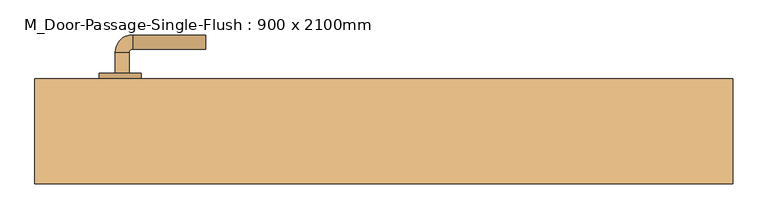
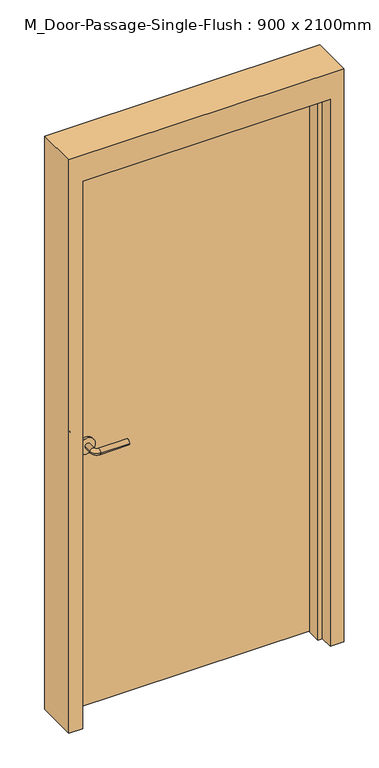
"""IFC4 building model written with IfcOpenShell, lengths in millimetres: door geometry, M_Door-Passage-Single-Flush : 900 x 2100mm."""

from ifc_helpers import new_model, si_unit, point, frame, frame_2d, origin, origin_with_axes, place, context, project, spatial, polyline, circle_curve, ellipse_curve, trimmed, segment, composite_curve, outline, extrude, faceted_brep, source, transform, mapped, element, save
from ifc_brep_helpers import plane_surface, cylinder_surface, revolved_surface, advanced_brep


def m_door_passage_single_flush_900_x_2100mm_f70d95c9(model_context):
    return source(origin(), model_context, "Body", "SolidModel", [
        advanced_brep(
        [(-384.990625, 3.35, 1000.0), (-364.990625, 3.35, 1000.0), (-364.990625, -26.65, 1000.0), (-384.990625, -26.65, 1000.0), (-359.990625, -31.65, 1000.0), (-359.990625, -51.65, 1000.0), (-254.990625, -51.65, 1000.0), (-254.990625, -31.65, 1000.0)],
        [
            (0, 1, circle_curve(frame((-374.990625, 3.35, 1000.0), z_axis=(0.0, 1.0, 0.0), x_axis=(1.0, 0.0, 0.0)), 10.0)),
            (1, 0, circle_curve(frame((-374.990625, 3.35, 1000.0), z_axis=(0.0, 1.0, 0.0), x_axis=(1.0, 0.0, 0.0)), 10.0)),
            (1, 2),
            (2, 3, circle_curve(frame((-374.990625, -26.65, 1000.0), z_axis=(0.0, 1.0, 0.0), x_axis=(1.0, 0.0, 0.0)), 10.0)),
            (3, 0),
            (3, 2, circle_curve(frame((-374.990625, -26.65, 1000.0), z_axis=(0.0, 1.0, 0.0), x_axis=(1.0, 0.0, 0.0)), 10.0)),
            (4, 5, circle_curve(frame((-359.990625, -41.65, 1000.0), z_axis=(-1.0, 0.0, 0.0), x_axis=(0.0, 1.0, 0.0)), 10.0)),
            (5, 3, circle_curve(frame((-359.990625, -26.65, 1000.0), z_axis=(0.0, 0.0, -1.0), x_axis=(-1.0, 0.0, 0.0)), 25.0)),
            (2, 4, circle_curve(frame((-359.990625, -26.65, 1000.0), z_axis=(0.0, 0.0, 1.0), x_axis=(-1.0, 0.0, 0.0)), 5.0)),
            (5, 4, circle_curve(frame((-359.990625, -41.65, 1000.0), z_axis=(-1.0, 0.0, 0.0), x_axis=(0.0, 1.0, 0.0)), 10.0)),
            (6, 7, circle_curve(frame((-254.990625, -41.65, 1000.0), z_axis=(1.0, 0.0, 0.0), x_axis=(0.0, 1.0, 0.0)), 10.0)),
            (7, 6, circle_curve(frame((-254.990625, -41.65, 1000.0), z_axis=(1.0, 0.0, 0.0), x_axis=(0.0, 1.0, 0.0)), 10.0)),
            (4, 7),
            (6, 5),
        ],
        [
            plane_surface(frame((-374.990625, 3.35, 1000.0), z_axis=(0.0, 1.0, 0.0), x_axis=(0.0, 0.0, 1.0))),
            cylinder_surface(frame((-374.990625, 3.35, 1000.0), z_axis=(0.0, 1.0, 0.0), x_axis=(1.0, 0.0, 0.0)), 10.0),
            revolved_surface(trimmed(ellipse_curve(frame((-374.990625, -26.65, 1000.0), z_axis=(0.0, -1.0, 0.0), x_axis=(1.0, 0.0, 0.0)), 10.0, 10.0), [point((-384.990625, -26.65, 1000.0))], [point((-364.990625, -26.65, 1000.0))], True, "CARTESIAN"), (-359.990625, -26.65, 1000.0), (0.0, 0.0, -1.0)),
            revolved_surface(trimmed(ellipse_curve(frame((-374.990625, -26.65, 1000.0), z_axis=(0.0, -1.0, 0.0), x_axis=(1.0, 0.0, 0.0)), 10.0, 10.0), [point((-364.990625, -26.65, 1000.0))], [point((-384.990625, -26.65, 1000.0))], True, "CARTESIAN"), (-359.990625, -26.65, 1000.0), (0.0, 0.0, -1.0)),
            plane_surface(frame((-254.990625, -41.65, 1000.0), z_axis=(1.0, 0.0, 0.0), x_axis=(0.0, 0.0, 1.0))),
            cylinder_surface(frame((-359.990625, -41.65, 1000.0), z_axis=(-1.0, 0.0, 0.0), x_axis=(0.0, 1.0, 0.0)), 10.0),
        ],
        [
            (0, [[1, 2]]),
            (1, [[3, 4, 5, -2]]),
            (1, [[-5, 6, -3, -1]]),
            (2, [[7, 8, -4, 9]]),
            (3, [[10, -9, -6, -8]]),
            (4, [[11, 12]]),
            (5, [[13, -11, 14, -7]]),
            (5, [[-14, -12, -13, -10]]),
        ],
    ),
        extrude(outline(composite_curve([segment(trimmed(circle_curve(frame_2d((1000.0, -377.490625)), 30.0), [point((1000.0, -407.490625))], [point((1000.0, -347.490625))], False, "CARTESIAN"), True, "CONTINUOUS"), segment(trimmed(circle_curve(frame_2d((1000.0, -377.490625)), 30.0), [point((1000.0, -347.490625))], [point((1000.0, -407.490625))], False, "CARTESIAN"), True, "CONTINUOUS")], self_intersect=False)), frame((0.0, 3.35, 0.0), z_axis=(0.0, 1.0, 0.0), x_axis=(0.0, 0.0, 1.0)), (0.0, 0.0, 1.0), 8.0),
        advanced_brep(
        [(-384.990625, 64.35, 1000.0), (-364.990625, 64.35, 1000.0), (-384.990625, 94.35, 1000.0), (-364.990625, 94.35, 1000.0), (-359.990625, 99.35, 1000.0), (-359.990625, 119.35, 1000.0), (-254.990625, 119.35, 1000.0), (-254.990625, 99.35, 1000.0)],
        [
            (0, 1, circle_curve(frame((-374.990625, 64.35, 1000.0), z_axis=(0.0, -1.0, 0.0), x_axis=(1.0, 0.0, 0.0)), 10.0)),
            (1, 0, circle_curve(frame((-374.990625, 64.35, 1000.0), z_axis=(0.0, -1.0, 0.0), x_axis=(1.0, 0.0, 0.0)), 10.0)),
            (0, 2),
            (2, 3, circle_curve(frame((-374.990625, 94.35, 1000.0), z_axis=(0.0, -1.0, 0.0), x_axis=(1.0, 0.0, 0.0)), 10.0)),
            (3, 1),
            (3, 2, circle_curve(frame((-374.990625, 94.35, 1000.0), z_axis=(0.0, -1.0, 0.0), x_axis=(1.0, 0.0, 0.0)), 10.0)),
            (4, 3, circle_curve(frame((-359.990625, 94.35, 1000.0), z_axis=(0.0, 0.0, 1.0), x_axis=(-1.0, 0.0, 0.0)), 5.0)),
            (2, 5, circle_curve(frame((-359.990625, 94.35, 1000.0), z_axis=(0.0, 0.0, -1.0), x_axis=(-1.0, 0.0, 0.0)), 25.0)),
            (5, 4, circle_curve(frame((-359.990625, 109.35, 1000.0), z_axis=(-1.0, 0.0, 0.0), x_axis=(0.0, -1.0, 0.0)), 10.0)),
            (4, 5, circle_curve(frame((-359.990625, 109.35, 1000.0), z_axis=(-1.0, 0.0, 0.0), x_axis=(0.0, -1.0, 0.0)), 10.0)),
            (6, 7, circle_curve(frame((-254.990625, 109.35, 1000.0), z_axis=(1.0, 0.0, 0.0), x_axis=(0.0, -1.0, 0.0)), 10.0)),
            (7, 6, circle_curve(frame((-254.990625, 109.35, 1000.0), z_axis=(1.0, 0.0, 0.0), x_axis=(0.0, -1.0, 0.0)), 10.0)),
            (5, 6),
            (7, 4),
        ],
        [
            plane_surface(frame((-374.990625, 64.35, 1000.0), z_axis=(0.0, -1.0, 0.0), x_axis=(0.0, 0.0, 1.0))),
            cylinder_surface(frame((-374.990625, 64.35, 1000.0), z_axis=(0.0, -1.0, 0.0), x_axis=(1.0, 0.0, 0.0)), 10.0),
            revolved_surface(trimmed(ellipse_curve(frame((-374.990625, 94.35, 1000.0), z_axis=(0.0, -1.0, 0.0), x_axis=(1.0, 0.0, 0.0)), 10.0, 10.0), [point((-384.990625, 94.35, 1000.0))], [point((-364.990625, 94.35, 1000.0))], True, "CARTESIAN"), (-359.990625, 94.35, 1000.0), (0.0, 0.0, -1.0)),
            revolved_surface(trimmed(ellipse_curve(frame((-374.990625, 94.35, 1000.0), z_axis=(0.0, -1.0, 0.0), x_axis=(1.0, 0.0, 0.0)), 10.0, 10.0), [point((-364.990625, 94.35, 1000.0))], [point((-384.990625, 94.35, 1000.0))], True, "CARTESIAN"), (-359.990625, 94.35, 1000.0), (0.0, 0.0, -1.0)),
            plane_surface(frame((-254.990625, 109.35, 1000.0), z_axis=(1.0, 0.0, 0.0), x_axis=(0.0, 0.0, 1.0))),
            cylinder_surface(frame((-359.990625, 109.35, 1000.0), z_axis=(-1.0, 0.0, 0.0), x_axis=(0.0, -1.0, 0.0)), 10.0),
        ],
        [
            (0, [[1, 2]]),
            (1, [[-1, 3, 4, 5]]),
            (1, [[-2, -5, 6, -3]]),
            (2, [[7, -4, 8, 9]]),
            (3, [[-8, -6, -7, 10]]),
            (4, [[11, 12]]),
            (5, [[-9, 13, -12, 14]]),
            (5, [[-10, -14, -11, -13]]),
        ],
    ),
        extrude(outline(composite_curve([segment(trimmed(circle_curve(frame_2d((1000.0, -377.490625)), 30.0), [point((1000.0, -407.490625))], [point((1000.0, -347.490625))], False, "CARTESIAN"), True, "CONTINUOUS"), segment(trimmed(circle_curve(frame_2d((1000.0, -377.490625)), 30.0), [point((1000.0, -347.490625))], [point((1000.0, -407.490625))], False, "CARTESIAN"), True, "CONTINUOUS")], self_intersect=False)), frame((0.0, 56.35, 0.0), z_axis=(0.0, 1.0, 0.0), x_axis=(0.0, 0.0, 1.0)), (0.0, 0.0, 1.0), 8.0),
        extrude(outline(polyline([(450.0, 11.35), (-450.0, 11.35), (-450.0, 56.35), (450.0, 56.35), (450.0, 11.35)])), origin_with_axes(), (0.0, 0.0, 1.0), 2100.0),
        faceted_brep([(450.0, 6.5875, 0.0), (450.0, 56.35, 0.0), (500.0, 56.35, 0.0), (500.0, -93.65, 0.0), (450.0, -93.65, 0.0), (450.0, -44.4375, 0.0), (434.125, -44.4375, 0.0), (434.125, 6.5875, 0.0), (450.0, 6.5875, 2100.0), (450.0, 56.35, 2100.0), (-450.0, 56.35, 2100.0), (-450.0, 56.35, 0.0), (-500.0, 56.35, 0.0), (-500.0, 56.35, 2200.0), (500.0, 56.35, 2200.0), (500.0, -93.65, 2200.0), (-500.0, -93.65, 2200.0), (-500.0, -93.65, 0.0), (-450.0, -93.65, 0.0), (-450.0, -93.65, 2100.0), (450.0, -93.65, 2100.0), (450.0, -44.4375, 2100.0), (-450.0, -44.4375, 2100.0), (-450.0, -44.4375, 0.0), (-434.125, -44.4375, 0.0), (-434.125, -44.4375, 2084.125), (434.125, -44.4375, 2084.125), (434.125, 6.5875, 2084.125), (-434.125, 6.5875, 2084.125), (-434.125, 6.5875, 0.0), (-450.0, 6.5875, 0.0), (-450.0, 6.5875, 2100.0)], [[[0, 1, 2, 3, 4, 5, 6, 7]], [[1, 0, 8, 9]], [[2, 1, 9, 10, 11, 12, 13, 14]], [[3, 2, 14, 15]], [[4, 3, 15, 16, 17, 18, 19, 20]], [[5, 4, 20, 21]], [[6, 5, 21, 22, 23, 24, 25, 26]], [[7, 6, 26, 27]], [[0, 7, 27, 28, 29, 30, 31, 8]], [[9, 8, 31, 10]], [[20, 19, 22, 21]], [[26, 25, 28, 27]], [[12, 11, 30, 29, 24, 23, 18, 17]], [[11, 10, 31, 30]], [[13, 12, 17, 16]], [[19, 18, 23, 22]], [[25, 24, 29, 28]], [[15, 14, 13, 16]]]),
    ])


if __name__ == "__main__":
    model = new_model("IFC4")
    model_context = context("Model", 3, world=origin())
    ifc_project = project(units=[si_unit("LENGTHUNIT", "METRE", prefix="MILLI")], contexts=[model_context])
    site = spatial("IfcSite", under=ifc_project)
    building = spatial("IfcBuilding", under=site)
    placement = place(None, origin())
    m_door_passage_single_flush_900_x_2100mm_shape = m_door_passage_single_flush_900_x_2100mm_f70d95c9(model_context)
    element("IfcDoor", 1, ObjectType="M_Door-Passage-Single-Flush : 900 x 2100mm", at=placement, inside=building, context=model_context, shape_type="MappedRepresentation", body=[
        mapped(m_door_passage_single_flush_900_x_2100mm_shape, transform((0.0, 0.0, 0.0), x_axis=(1.0, 0.0, 0.0), y_axis=(0.0, 1.0, 0.0), z_axis=(0.0, 0.0, 1.0))),
    ])
    save(model, "model.ifc")

# Revit data of these elements
# Type "M_Door-Passage-Single-Flush : 900 x 2100mm"
#   Type Mark = "38"
#   Analytic Construction = "Wooden"
#   Thickness = 45 mm
#   Thermal Resistance (R) = 0.455703 (m²·K)/W
#   Swing Angle [instance default] = 90.00°
#   Strike Height = 1000 mm
#   Rough Width [instance default] = 1000 mm
#   Rough Height [instance default] = 2200 mm
#   MF Opening Height [instance default] = 100 mm
#   MF Opening Width [instance default] = 100 mm
#   Inset Calculate [instance default] = 105 mm
#   Masonry Inset [instance default] = 25 mm
#   Height = 2100 mm
#   Width = 900 mm
#   Heat Transfer Coefficient (U) = 2.19465 W/(m²·K)
#   Masonry Frame Depth = 150 mm
#   Masonry Frame [instance default] = yes
#   Function = 1
#   Dry Wall Frame [instance default] = no
#   Panel Material = Wood - Birch
#   Frame Material = Metal - Paint Finish - Grey
#   Door Handle Material = Aluminum
#   Visual Light Transmittance = 0
#   Solar Heat Gain Coefficient = 0
#   Wall Closure = (empty or 0)
# Element 1 (IfcDoor, "M_Door-Passage-Single-Flush : 900 x 2100mm")
#   Materials on its faces: "Aluminum", "Metal - Paint Finish - Grey", "Wood - Birch"
# Materials
#   "Wood - Birch": class "Wood", colour RGB 173 132 96, transparency 0, Cost = 0
#   "Metal - Paint Finish - Grey": class "Paint", colour RGB 178 178 178, transparency 0, Cost = 0
#   "Aluminum": class "Metal", colour RGB 244 245 246, transparency 0, Description = "Aluminum 6061", Cost = 0
